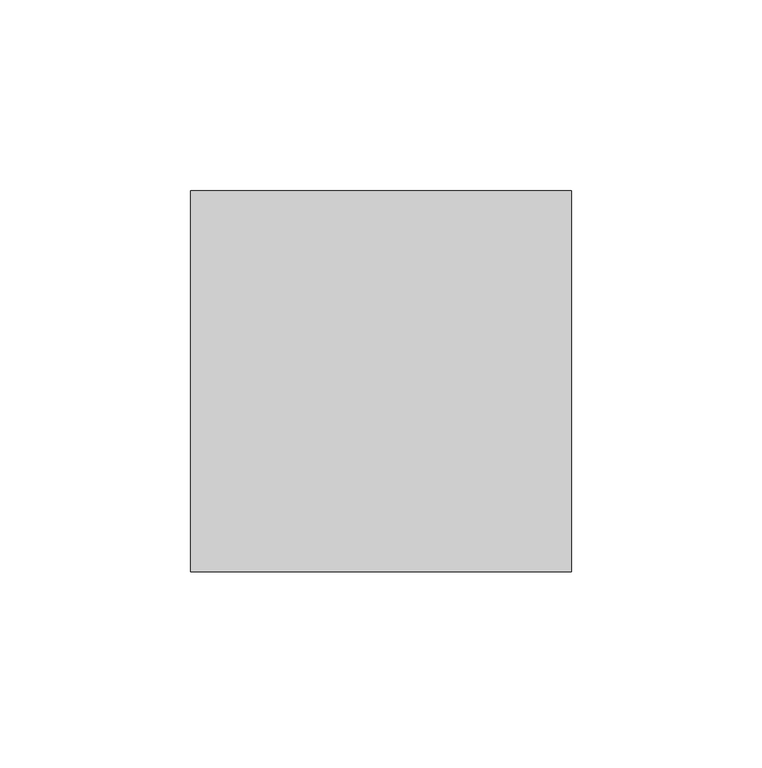
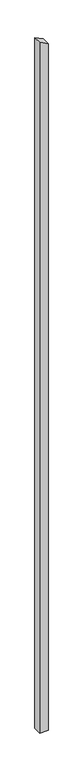
"""IFC4 building model written with IfcOpenShell, lengths in millimetres: column geometry, Holzstütze : Holzstütze."""

from ifc_helpers import new_model, si_unit, frame, origin, place, context, project, spatial, polyline, outline, extrude, source, transform, mapped, element, save


def column_49ea4e92(model_context):
    return source(origin(), model_context, "Body", "SweptSolid", [
        extrude(outline(polyline([(-500.0, 170469.1702308), (-500.0, 170569.1702308), (8245.522848, 170569.1702308), (8296.4753929, 170469.1702308), (-500.0, 170469.1702308)])), frame((0.0, 47884.7962965, 0.0), z_axis=(0.0, 1.0, 0.0), x_axis=(0.0, 0.0, 1.0)), (0.0, 0.0, 1.0), 100.0),
    ])


if __name__ == "__main__":
    model = new_model("IFC4")
    model_context = context("Model", 3, world=origin())
    ifc_project = project(units=[si_unit("LENGTHUNIT", "METRE", prefix="MILLI")], contexts=[model_context])
    site = spatial("IfcSite", under=ifc_project)
    building = spatial("IfcBuilding", under=site)
    placement = place(None, origin())
    column_shape = column_49ea4e92(model_context)
    element("IfcColumn", 1, ObjectType="Holzstütze : Holzstütze", at=placement, inside=building, context=model_context, shape_type="MappedRepresentation", body=[
        mapped(column_shape, transform((0.0, 0.0, 0.0), x_axis=(1.0, 0.0, 0.0), y_axis=(0.0, 1.0, 0.0), z_axis=(0.0, 0.0, 1.0))),
    ])
    save(model, "model.ifc")

# Revit data of these elements
# Type "Holzstütze : Holzstütze"
#   Abrechnungsart = "m"
#   Allright_Bauteil_ID = "0152St 0000143546"
#   Bezeichnung = "Holzstütze"
#   Codetext = "ST-HOLZ\\"
#   Gewerk = "Zimmer- und Holzbauarbeiten"
#   Material = "Holz"
#   Objektname = "Stütze"
#   NameOverride = "Holzstütze"
#   Reference = "Holzstütze"
#   Status = "NEW"
#   ThermalTransmittance = 0.0000 BTU/(h·ft²·°F)
#   Roll = 0.00°
#   Slope = 0.00°
#   2D Interaktion = yes
#   IsExternal = yes
#   LoadBearing = yes
# Element 1 (IfcColumn, "Holzstütze : Holzstütze")
#   Materials on its faces: "holzschalung"
# Materials
#   "holzschalung": class "Unassigned", colour RGB 128 128 128, transparency 0
